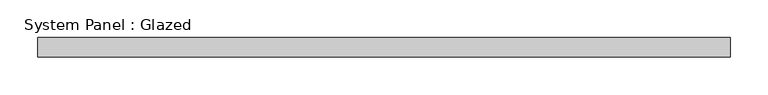
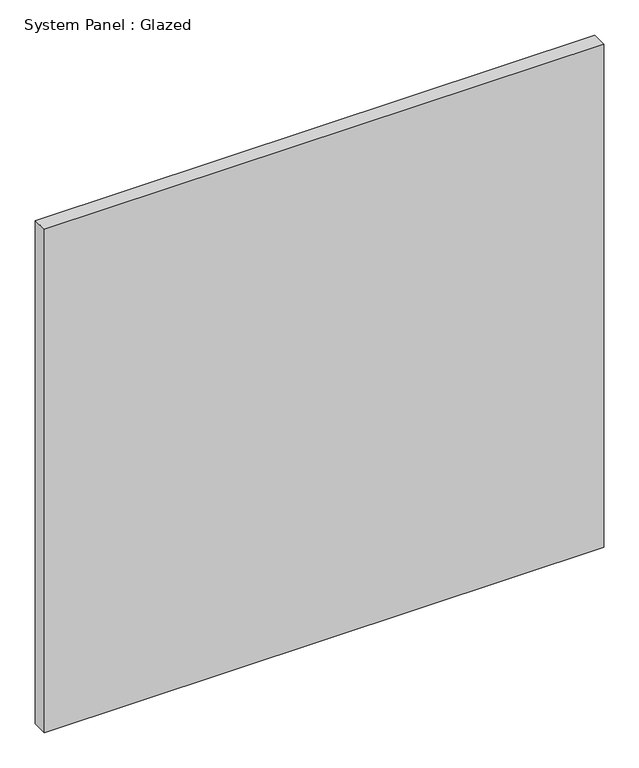
"""IFC4 building model written with IfcOpenShell, lengths in millimetres: plate geometry, System Panel : Glazed."""

from ifc_helpers import new_model, si_unit, origin, origin_with_axes, place, context, project, spatial, polyline, outline, extrude, source, transform, mapped, element, save


def system_panel_glazed_63e32c76(model_context):
    return source(origin(), model_context, "Body", "SweptSolid", [
        extrude(outline(polyline([(457.2, 19.05), (-457.2, 19.05), (-457.2, 44.45), (457.2, 44.45), (457.2, 19.05)])), origin_with_axes(), (0.0, 0.0, 1.0), 869.95),
    ])


if __name__ == "__main__":
    model = new_model("IFC4")
    model_context = context("Model", 3, world=origin())
    ifc_project = project(units=[si_unit("LENGTHUNIT", "METRE", prefix="MILLI")], contexts=[model_context])
    site = spatial("IfcSite", under=ifc_project)
    building = spatial("IfcBuilding", under=site)
    placement = place(None, origin())
    system_panel_glazed_shape = system_panel_glazed_63e32c76(model_context)
    element("IfcPlate", 1, ObjectType="System Panel : Glazed", at=placement, inside=building, context=model_context, shape_type="MappedRepresentation", body=[
        mapped(system_panel_glazed_shape, transform((0.0, 0.0, 0.0), x_axis=(1.0, 0.0, 0.0), y_axis=(0.0, 1.0, 0.0), z_axis=(0.0, 0.0, 1.0))),
    ])
    save(model, "model.ifc")

# Revit data of these elements
# Element 1 (IfcPlate, "System Panel : Glazed")
#   Materials on its faces: "Glass"
# Materials
#   "Glass": class "Glass", colour RGB 0 128 192, transparency 0.75
